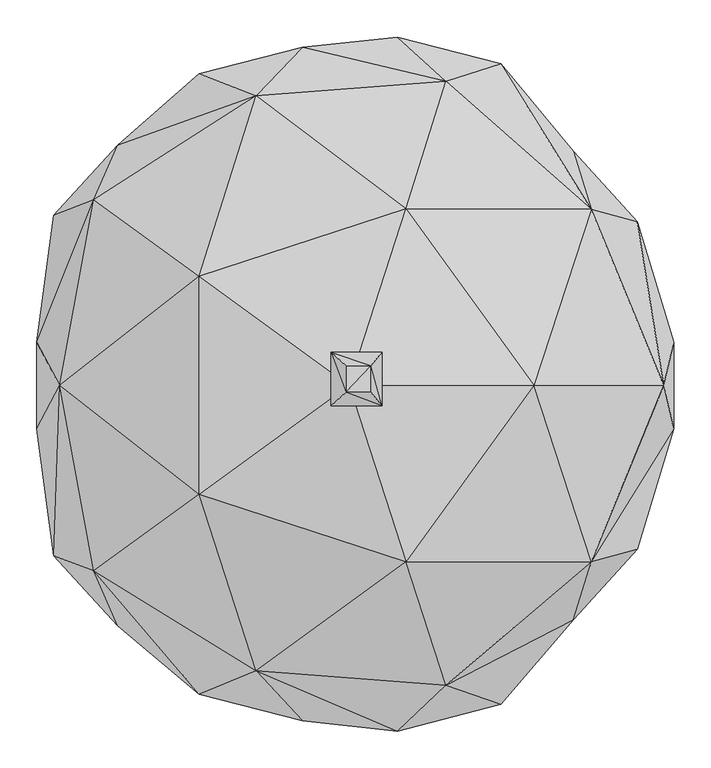
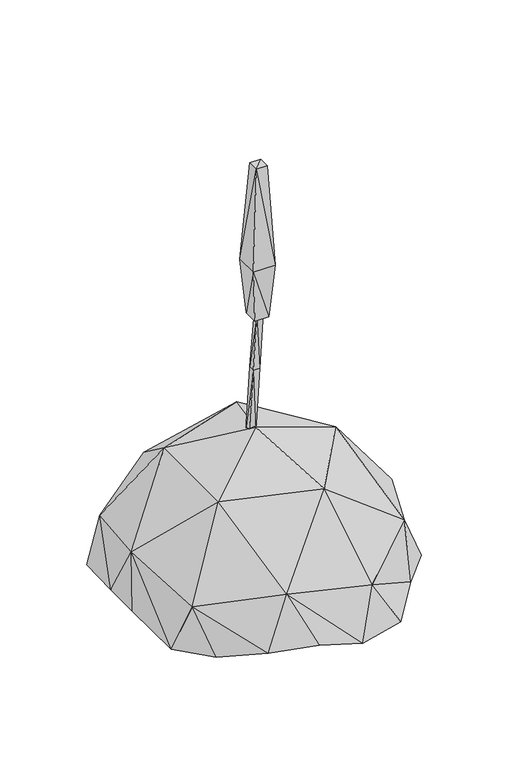
"""IFC4 building model written with IfcOpenShell, lengths in millimetres: geographic element geometry, Enscape AssetDefinition - Asparagaceae 002 Desert Spoon : Enscape AssetDefinition - Asparagaceae 002 Desert Spoon."""

from ifc_helpers import new_model, si_unit, origin, place, context, project, spatial, faceted_brep, source, transform, mapped, element, save


def geographic_element_90c88f6b(model_context):
    return source(origin(), model_context, "Body", "Brep", [
        faceted_brep([(77.3755834, 231.930241, 497.5196719), (-0.1228665, -6.5854914, 584.869504), (250.6673932, -6.5854914, 497.5196719), (-203.0164748, 140.8253163, 497.5196719), (-203.016445, -153.9963335, 497.5196719), (77.3756281, -245.1011837, 497.5196719), (328.165859, 231.930241, 307.4840605), (-125.5180389, 385.0497603, 307.4840605), (131.7253709, 404.9103856, 261.5615726), (-391.3793266, -6.5855347, 307.4840605), (-345.3060985, 244.2047596, 261.5615726), (-202.8535455, 414.6253765, 157.2964489), (-62.7697259, 450.901866, 157.296434), (-312.659651, 318.3333576, 127.2263825), (65.7490641, 464.4800723, 127.2263974), (205.8328837, 428.203553, 127.2263825), (-0.1228734, 173.6139804, -5.6e-06), (-181.9830239, 139.1989589, -4.6e-06), (-399.2362618, 223.3601809, 127.2263974), (-294.3788469, 49.0991697, -1.7e-06), (-0.1228542, -6.5854951, 0.0), (181.7373335, 139.1989291, -4.6e-06), (303.9745688, 309.9415898, 157.296434), (294.1331267, 49.099192, -1.7e-06), (390.5511796, 214.9684429, 157.2964489), (426.5470505, -6.5854914, 261.5615726), (439.7023916, 51.9014038, 127.2263974), (294.1331267, -62.2701943, 1.7e-06), (439.7023916, -65.4918104, 127.2263974), (328.1658888, -245.1011986, 307.4840605), (131.7254454, -412.3726487, 261.5615726), (390.5511796, -228.5588086, 157.2964489), (303.9746284, -323.5318959, 157.2964936), (181.7374229, -152.3699164, 4.6e-06), (205.8330327, -437.8910959, 127.2263974), (-125.5179644, -392.5120533, 307.4840605), (65.749228, -474.167645, 127.2263974), (-345.3060687, -257.3758066, 261.5615726), (-62.7695397, -460.5894387, 157.2964936), (-202.853471, -424.312979, 157.2964936), (-0.1226974, -186.7849529, 5.6e-06), (-181.9829941, -152.3699462, 4.6e-06), (-312.6596212, -331.9238126, 127.2263974), (-399.2361724, -236.9506061, 127.2263974), (-294.3788171, -62.2701868, 1.7e-06), (-422.2543836, -65.4918328, 157.296434), (-422.2543836, 51.9013554, 157.296434)], [[[0, 1, 2]], [[3, 1, 0]], [[4, 1, 3]], [[5, 1, 4]], [[2, 1, 5]], [[2, 6, 0]], [[0, 7, 3]], [[8, 0, 6]], [[7, 0, 8]], [[3, 9, 4]], [[10, 3, 7]], [[9, 3, 10]], [[11, 7, 12]], [[8, 12, 7]], [[7, 13, 10]], [[13, 7, 11]], [[14, 8, 15]], [[6, 15, 8]], [[12, 8, 14]], [[14, 16, 12]], [[17, 12, 16]], [[12, 17, 11]], [[11, 17, 13]], [[18, 10, 13]], [[19, 13, 17]], [[13, 19, 18]], [[20, 17, 16]], [[20, 19, 17]], [[20, 16, 21]], [[16, 15, 21]], [[15, 16, 14]], [[22, 21, 15]], [[15, 6, 22]], [[20, 21, 23]], [[21, 24, 23]], [[24, 21, 22]], [[22, 6, 24]], [[6, 2, 25]], [[25, 24, 6]], [[26, 23, 24]], [[24, 25, 26]], [[20, 23, 27]], [[26, 27, 23]], [[26, 25, 28]], [[26, 28, 27]], [[25, 2, 29]], [[29, 28, 25]], [[5, 29, 2]], [[29, 5, 30]], [[31, 29, 32]], [[30, 32, 29]], [[28, 29, 31]], [[31, 27, 28]], [[32, 27, 31]], [[20, 27, 33]], [[27, 32, 33]], [[34, 33, 32]], [[32, 30, 34]], [[30, 5, 35]], [[34, 30, 36]], [[35, 36, 30]], [[4, 35, 5]], [[35, 4, 37]], [[38, 35, 39]], [[37, 39, 35]], [[36, 35, 38]], [[38, 40, 36]], [[33, 36, 40]], [[36, 33, 34]], [[20, 33, 40]], [[20, 40, 41]], [[40, 39, 41]], [[39, 40, 38]], [[42, 41, 39]], [[39, 37, 42]], [[37, 4, 9]], [[42, 37, 43]], [[9, 43, 37]], [[43, 41, 42]], [[20, 41, 44]], [[41, 43, 44]], [[45, 44, 43]], [[43, 9, 45]], [[45, 9, 46]], [[10, 46, 9]], [[46, 44, 45]], [[20, 44, 19]], [[44, 46, 19]], [[18, 19, 46]], [[46, 10, 18]]]),
        faceted_brep([(32.1177915, 25.0110235, 949.3535161), (-11.6653657, 25.0110198, 949.3535161), (-24.1568722, 38.2373109, 1124.0200996), (-11.6653657, -21.3476103, 949.3535161), (32.1177915, -21.3476103, 949.3535161), (-24.1568778, -34.5739201, 1124.0200996), (44.6093008, 38.2373072, 1124.0200996), (44.6092971, -34.5739312, 1124.0200996), (-4.1842223, -16.2918922, 1447.7174282), (30.0490744, 19.9551284, 1447.7174282), (30.0490744, -16.2918922, 1447.7174282), (-4.1842223, 19.9551284, 1447.7174282)], [[[0, 1, 2]], [[3, 1, 4]], [[5, 2, 1]], [[4, 1, 0]], [[5, 1, 3]], [[4, 0, 6]], [[0, 2, 6]], [[5, 3, 4]], [[5, 4, 7]], [[4, 6, 7]], [[5, 7, 8]], [[8, 2, 5]], [[7, 6, 9]], [[8, 7, 10]], [[7, 9, 10]], [[6, 2, 9]], [[10, 9, 8]], [[8, 9, 11]], [[9, 2, 11]], [[8, 11, 2]]]),
        faceted_brep([(5.8008027, 20.3128941, 562.6442432), (-15.9671251, 20.3128941, 562.6442432), (-5.9760879, 17.4094476, 773.27317), (-15.9671251, 3.0921863, 562.6442432), (5.8008051, 3.092184, 562.6442432), (-5.9760879, -2.8190413, 773.2731104), (14.8979994, 17.4094476, 773.27317), (2.741921, -7.0615048, 957.0643306), (2.741921, 8.2554398, 957.0643306), (14.8980012, -2.8190413, 773.2731104), (22.8360649, 8.2554379, 957.0643306), (22.8360649, -7.0615094, 957.0643306)], [[[0, 1, 2]], [[3, 1, 4]], [[5, 2, 1]], [[4, 1, 0]], [[5, 1, 3]], [[4, 0, 6]], [[0, 2, 6]], [[7, 8, 2]], [[6, 2, 8]], [[7, 2, 5]], [[5, 3, 4]], [[5, 9, 7]], [[5, 4, 9]], [[4, 6, 9]], [[9, 6, 10]], [[6, 8, 10]], [[7, 10, 8]], [[11, 10, 7]], [[7, 9, 11]], [[9, 10, 11]]]),
    ])


if __name__ == "__main__":
    model = new_model("IFC4")
    model_context = context("Model", 3, world=origin())
    ifc_project = project(units=[si_unit("LENGTHUNIT", "METRE", prefix="MILLI")], contexts=[model_context])
    site = spatial("IfcSite", under=ifc_project)
    building = spatial("IfcBuilding", under=site)
    placement = place(None, origin())
    geographic_element_shape = geographic_element_90c88f6b(model_context)
    element("IfcGeographicElement", 1, ObjectType="Enscape AssetDefinition - Asparagaceae 002 Desert Spoon : Enscape AssetDefinition - Asparagaceae 002 Desert Spoon", at=placement, inside=building, context=model_context, shape_type="MappedRepresentation", body=[
        mapped(geographic_element_shape, transform((0.0, 0.0, 0.0), x_axis=(1.0, 0.0, 0.0), y_axis=(0.0, 1.0, 0.0), z_axis=(0.0, 0.0, 1.0))),
    ])
    save(model, "model.ifc")

# Revit data of these elements
# Type "Enscape AssetDefinition - Asparagaceae 002 Desert Spoon : Enscape AssetDefinition - Asparagaceae 002 Desert Spoon"
#   EnscapeAssetSource = "REMOTE"
#   EnscapeAssetId = "3817e39e-d8b9-4ce2-b22c-b5864509c2b9"
#   Height = 1.447717 m
#   EnscapeNativeAssetHeight = 1.447717 m
#   Default Elevation = 0
